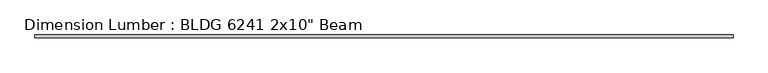
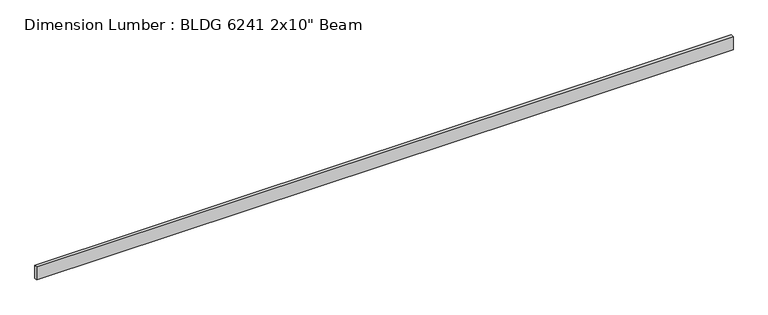
"""IFC4 building model written with IfcOpenShell, lengths in millimetres: beam geometry."""

from ifc_helpers import new_model, si_unit, frame, origin, place, context, project, spatial, polyline, outline, extrude, source, transform, mapped, element, save


def beam_bcf194da(model_context):
    return source(origin(), model_context, "Body", "SweptSolid", [
        extrude(outline(polyline([(6302.375, 25.4), (6302.375, -25.4), (-6429.375, -25.4), (-6429.375, 25.4), (6302.375, 25.4)])), frame((0.0, 0.0, -127.0), z_axis=(0.0, 0.0, 1.0), x_axis=(1.0, 0.0, 0.0)), (0.0, 0.0, 1.0), 254.0),
    ])


if __name__ == "__main__":
    model = new_model("IFC4")
    model_context = context("Model", 3, world=origin())
    ifc_project = project(units=[si_unit("LENGTHUNIT", "METRE", prefix="MILLI")], contexts=[model_context])
    site = spatial("IfcSite", under=ifc_project)
    building = spatial("IfcBuilding", under=site)
    placement = place(None, origin())
    beam_shape = beam_bcf194da(model_context)
    element("IfcBeam", 1, ObjectType="Dimension Lumber : BLDG 6241 2x10\" Beam", at=placement, inside=building, context=model_context, shape_type="MappedRepresentation", body=[
        mapped(beam_shape, transform((0.0, 0.0, 0.0), x_axis=(1.0, 0.0, 0.0), y_axis=(0.0, 1.0, 0.0), z_axis=(0.0, 0.0, 1.0))),
    ])
    save(model, "model.ifc")

# Revit data of these elements
# Type "Dimension Lumber : BLDG 6241 2x10\" Beam"
#   Assembly Code = "B10"
#   A = 0.273472 SF
#   Length [instance default] = 5' - 0"
#   b = 0' - 2"
#   d = 0' - 10"
#   Structural Material [instance default] = Softwood, Lumber
# Element 1 (IfcBeam, "Dimension Lumber : BLDG 6241 2x10\" Beam")
#   Materials on its faces: "Softwood, Lumber"
# Materials
#   "Softwood, Lumber": class "Wood", colour RGB 223 192 134, transparency 0, Description = "Pinus Echinata", Cost = 0
